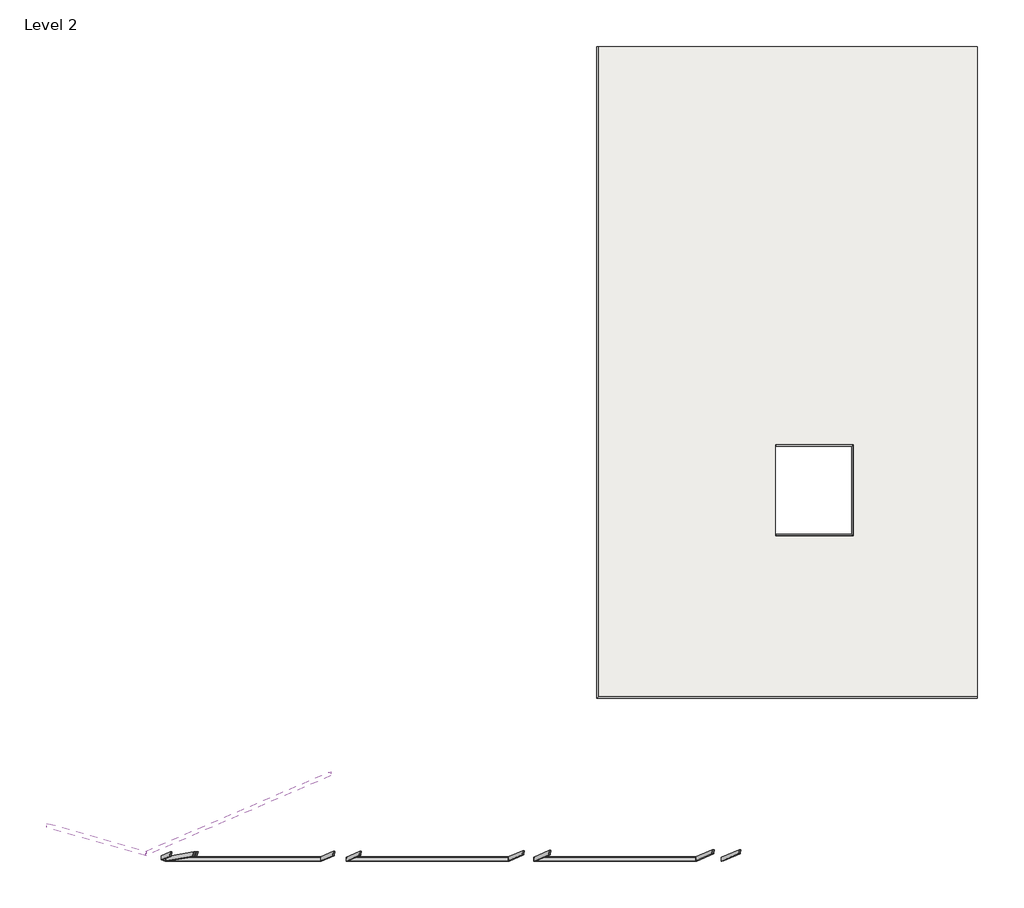
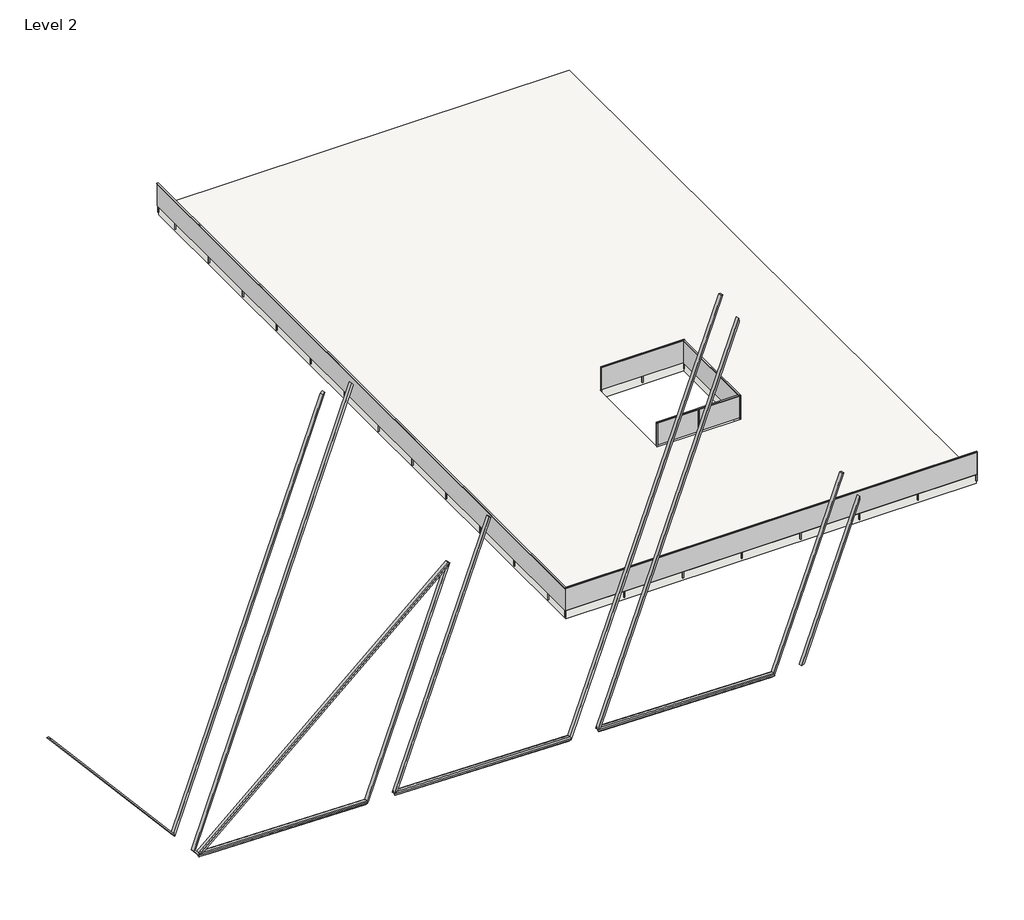
# One storey: 18 members, 2 railings, 1 slab.
"""IFC4 building model written with IfcOpenShell, lengths in millimetres."""

import ifcopenshell
import ifcopenshell.guid

model = None  # the IFC model being written
_history = None  # IfcOwnerHistory: only IFC2X3 demands one
_inside = {}  # id of a spatial element -> (the spatial element, [elements in it])
_under = {}  # id of a project, library or spatial element -> (it, [spatial elements below it])
_declared = {}  # id of a project -> (the project, [libraries it declares])
_typed = {}  # id of a type object -> (the type object, [elements of that type])
_made_of = {}  # id of a material, layer set ... -> (it, [elements and type objects made of it])


def new_model(schema):
    """Start an empty IFC model of exactly this schema.

    Asked for "IFC4X3", IfcOpenShell would pick the latest addendum, in which some entities
    have other attributes; the version numbers below select the first issue.
    IFC2X3 requires an IfcOwnerHistory on every rooted entity: one is made here for all.
    """
    global model, _history
    if schema == "IFC4X3":
        model = ifcopenshell.file(schema_version=(4, 3, 0, 0))
    else:
        model = ifcopenshell.file(schema=schema)
    _inside.clear()
    _under.clear()
    _declared.clear()
    _typed.clear()
    _made_of.clear()
    _history = None
    if model.schema == "IFC2X3":
        org = make("IfcOrganization", Name="unknown")
        user = make(
            "IfcPersonAndOrganization",
            ThePerson=make("IfcPerson", FamilyName="unknown"),
            TheOrganization=org,
        )
        app = make(
            "IfcApplication",
            ApplicationDeveloper=org,
            Version="unknown",
            ApplicationFullName="unknown",
            ApplicationIdentifier="unknown",
        )
        _history = make(
            "IfcOwnerHistory",
            OwningUser=user,
            OwningApplication=app,
            ChangeAction="ADDED",
            CreationDate=0,
        )
    return model


def make(cls, **values):
    """One entity of the class cls with the attributes given. An attribute that is None is left unset."""
    return model.create_entity(
        cls, **{name: value for name, value in values.items() if value is not None}
    )


def rooted(cls, **values):
    """An entity with a GlobalId (a new one), such as an element, a storey or a relation."""
    return make(cls, GlobalId=ifcopenshell.guid.new(), OwnerHistory=_history, **values)


def si_unit(unit_type, name, prefix=None):
    """IfcSIUnit, for example si_unit("LENGTHUNIT", "METRE", prefix="MILLI")."""
    return make("IfcSIUnit", UnitType=unit_type, Prefix=prefix, Name=name)


def assignment(units):
    """IfcUnitAssignment: the units of a project."""
    return None if units is None else make("IfcUnitAssignment", Units=units)


def point(xyz):
    """IfcCartesianPoint."""
    return None if xyz is None else make("IfcCartesianPoint", Coordinates=xyz)


def direction(xyz):
    """IfcDirection."""
    return None if xyz is None else make("IfcDirection", DirectionRatios=xyz)


def frame(location, z_axis=None, x_axis=None):
    """IfcAxis2Placement3D, a coordinate frame: its origin and axes. An axis left out is left unset."""
    return make(
        "IfcAxis2Placement3D",
        Location=point(location),
        Axis=direction(z_axis),
        RefDirection=direction(x_axis),
    )


def origin():
    """The frame at (0, 0, 0) with its axes left unset."""
    return frame((0.0, 0.0, 0.0))


def place(relative_to, where):
    """IfcLocalPlacement: puts the frame where relative to a parent placement (None: the world)."""
    return make(
        "IfcLocalPlacement", PlacementRelTo=relative_to, RelativePlacement=where
    )


def context(
    kind, dimensions, precision=None, world=None, true_north=None, identifier=None
):
    """IfcGeometricRepresentationContext, for example the 3D "Model" context."""
    return make(
        "IfcGeometricRepresentationContext",
        ContextIdentifier=identifier,
        ContextType=kind,
        CoordinateSpaceDimension=dimensions,
        Precision=precision,
        WorldCoordinateSystem=world,
        TrueNorth=true_north,
    )


def project(units=None, contexts=None):
    """IfcProject with its units and contexts."""
    return rooted(
        "IfcProject",
        Name="project",
        RepresentationContexts=contexts,
        UnitsInContext=assignment(units),
    )


def spatial(cls, under=None, at=None, **own):
    """A site, building, storey or space (cls), placed at a placement, below another one or the project."""
    s = rooted(cls, ObjectPlacement=at, **own)
    if under is not None:
        _under.setdefault(under.id(), (under, []))[1].append(s)
    return s


def polyline(points):
    """IfcPolyline through the points."""
    return make("IfcPolyline", Points=[point(p) for p in points])


def outline(outer, holes=None, kind="AREA"):
    """IfcArbitraryClosedProfileDef: a profile drawn as a closed curve; with holes, ...WithVoids."""
    if holes is None:
        return make("IfcArbitraryClosedProfileDef", ProfileType=kind, OuterCurve=outer)
    return make(
        "IfcArbitraryProfileDefWithVoids",
        ProfileType=kind,
        OuterCurve=outer,
        InnerCurves=holes,
    )


def extrude(swept, where, along, depth):
    """IfcExtrudedAreaSolid: the profile swept, set in the frame where, extruded along a direction by depth."""
    return make(
        "IfcExtrudedAreaSolid",
        SweptArea=swept,
        Position=where,
        ExtrudedDirection=direction(along),
        Depth=depth,
    )


def faces_of(points, faces, orient=None, outer=None):
    """IfcFace entities. A face is a list of loops; a loop is a list of indices into points, from 0.

    orient and outer hold one flag for each loop. By default every Orientation is true, the
    first loop of a face is its IfcFaceOuterBound and the others are IfcFaceBound.
    """
    made = []
    for i, loops in enumerate(faces):
        bounds = []
        for j, loop in enumerate(loops):
            is_outer = j == 0 if outer is None else outer[i][j]
            bounds.append(
                make(
                    "IfcFaceOuterBound" if is_outer else "IfcFaceBound",
                    Bound=make("IfcPolyLoop", Polygon=[points[k] for k in loop]),
                    Orientation=True if orient is None else orient[i][j],
                )
            )
        made.append(make("IfcFace", Bounds=bounds))
    return made


def faceted_brep(points, faces, orient=None, outer=None, voids=None):
    """IfcFacetedBrep: a solid bounded by flat faces; with voids (closed shells), ...WithVoids."""
    shared = [point(p) for p in points]
    hull = make("IfcClosedShell", CfsFaces=faces_of(shared, faces, orient, outer))
    if voids is None:
        return make("IfcFacetedBrep", Outer=hull)
    return make(
        "IfcFacetedBrepWithVoids",
        Outer=hull,
        Voids=[
            make(cls, CfsFaces=faces_of(shared, fs, o, b)) for cls, fs, o, b in voids
        ],
    )


def shape(context_of_items, identifier, shape_type, items):
    """IfcShapeRepresentation: the items that make up one representation, for example the "Body"."""
    return make(
        "IfcShapeRepresentation",
        ContextOfItems=context_of_items,
        RepresentationIdentifier=identifier,
        RepresentationType=shape_type,
        Items=items,
    )


def source(mapping_origin, context_of_items, identifier, shape_type, items):
    """IfcRepresentationMap: a shape defined once, which mapped items show again and again."""
    return make(
        "IfcRepresentationMap",
        MappingOrigin=mapping_origin,
        MappedRepresentation=shape(context_of_items, identifier, shape_type, items),
    )


def transform(
    local_origin,
    x_axis=None,
    y_axis=None,
    z_axis=None,
    scale=None,
    scale2=None,
    scale3=None,
    uniform=True,
):
    """IfcCartesianTransformationOperator3D, or its non-uniform kind. x_axis, y_axis, z_axis: its Axis1, 2, 3."""
    if uniform:
        return make(
            "IfcCartesianTransformationOperator3D",
            Axis1=direction(x_axis),
            Axis2=direction(y_axis),
            LocalOrigin=point(local_origin),
            Scale=scale,
            Axis3=direction(z_axis),
        )
    return make(
        "IfcCartesianTransformationOperator3DnonUniform",
        Axis1=direction(x_axis),
        Axis2=direction(y_axis),
        LocalOrigin=point(local_origin),
        Scale=scale,
        Axis3=direction(z_axis),
        Scale2=scale2,
        Scale3=scale3,
    )


def mapped(mapping_source, mapping_target):
    """IfcMappedItem: shows the shape of a source again, moved by a transform."""
    return make(
        "IfcMappedItem", MappingSource=mapping_source, MappingTarget=mapping_target
    )


def made_of(thing, what):
    """Note that an element or type object is made of a material, layer set ...; save() writes the relation."""
    if what is not None:
        _made_of.setdefault(what.id(), (what, []))[1].append(thing)
    return thing


def element(
    cls,
    number,
    at=None,
    inside=None,
    cuts=None,
    type_object=None,
    material=None,
    context=None,
    identifier="Body",
    shape_type=None,
    held_by="IfcProductDefinitionShape",
    body=None,
    shapes=None,
    **own,
):
    """One element of the class cls, such as IfcWall. Its Tag is "e" and its number.

    at: its placement. inside: the storey or other place that contains it. cuts: it is an
    opening in that element (IfcRelVoidsElement). A single representation is given by context,
    identifier, shape_type and body (its items); several are given by shapes. held_by: the class
    of the entity that holds the representations. save() writes the other relations.
    """
    e = rooted(cls, Tag="e%d" % number, ObjectPlacement=at, **own)
    if body is not None:
        shapes = [shape(context, identifier, shape_type, body)]
    if shapes is not None:
        e.Representation = make(held_by, Representations=shapes)
    if inside is not None:
        _inside.setdefault(inside.id(), (inside, []))[1].append(e)
    if cuts is not None:
        rooted(
            "IfcRelVoidsElement", RelatingBuildingElement=cuts, RelatedOpeningElement=e
        )
    if type_object is not None:
        _typed.setdefault(type_object.id(), (type_object, []))[1].append(e)
    return made_of(e, material)


def aggregate(whole, parts):
    """IfcRelAggregates: a whole, such as a stair, and the parts it consists of."""
    return rooted("IfcRelAggregates", RelatingObject=whole, RelatedObjects=parts)


def save(model, path):
    """Write the relations noted so far, then the file.

    IfcRelAggregates (storeys below a building ...), IfcRelContainedInSpatialStructure (elements
    in a storey), IfcRelDefinesByType, IfcRelAssociatesMaterial and IfcRelDeclares: one each for
    every whole, place, type object, material and project.
    """
    for whole, parts in _under.values():
        aggregate(whole, parts)
    for where, things in _inside.values():
        rooted(
            "IfcRelContainedInSpatialStructure",
            RelatedElements=things,
            RelatingStructure=where,
        )
    for kind, things in _typed.values():
        rooted("IfcRelDefinesByType", RelatedObjects=things, RelatingType=kind)
    for what, things in _made_of.values():
        rooted("IfcRelAssociatesMaterial", RelatedObjects=things, RelatingMaterial=what)
    for by, libraries in _declared.values():
        rooted("IfcRelDeclares", RelatingContext=by, RelatedDefinitions=libraries)
    model.write(path)


def rectangular_mullion_50_x_150mm_45e6ae42(model_context):
    return source(origin(), model_context, "Body", "SweptSolid", [
        extrude(outline(polyline([(0.0, 0.0), (-213.5028682, -50.0), (-7489.7328456, -50.0), (-7519.6193703, 0.0), (0.0, 0.0)])), frame((0.0, -75.0, 0.0), z_axis=(0.0, 1.0, 0.0), x_axis=(0.0, 0.0, 1.0)), (0.0, 0.0, 1.0), 150.0),
    ])


def rectangular_mullion_50_x_150mm_7bc3959f(model_context):
    return source(origin(), model_context, "Body", "SweptSolid", [
        extrude(outline(polyline([(0.0, 0.0), (-25.8377402, -50.0), (-13921.2143035, -50.0), (-13951.1008282, 0.0), (0.0, 0.0)])), frame((0.0, -75.0, 0.0), z_axis=(0.0, 1.0, 0.0), x_axis=(0.0, 0.0, 1.0)), (0.0, 0.0, 1.0), 150.0),
    ])


def rectangular_mullion_50_x_150mm_85ac93d7(model_context):
    return source(origin(), model_context, "Body", "SweptSolid", [
        extrude(outline(polyline([(0.0, 0.0), (-25.8377402, -50.0), (-6312.9528574, -50.0), (-6342.8393821, 0.0), (0.0, 0.0)])), frame((0.0, -75.0, 0.0), z_axis=(0.0, 1.0, 0.0), x_axis=(0.0, 0.0, 1.0)), (0.0, 0.0, 1.0), 150.0),
    ])


def rectangular_mullion_50_x_150mm_72219edf(model_context):
    return source(origin(), model_context, "Body", "SweptSolid", [
        extrude(outline(polyline([(0.0, 0.0), (-83.6497392, -50.0), (-5243.3853965, -50.0), (-5340.1430845, 0.0), (0.0, 0.0)])), frame((0.0, -75.0, 0.0), z_axis=(0.0, 1.0, 0.0), x_axis=(0.0, 0.0, 1.0)), (0.0, 0.0, 1.0), 150.0),
    ])


def rectangular_mullion_50_x_150mm_d07257d7(model_context):
    return source(origin(), model_context, "Body", "SweptSolid", [
        extrude(outline(polyline([(0.0, 0.0), (-83.6497392, -50.0), (-8698.3621073, -50.0), (-8710.0715519, 0.0), (0.0, 0.0)])), frame((0.0, -75.0, 0.0), z_axis=(0.0, 1.0, 0.0), x_axis=(0.0, 0.0, 1.0)), (0.0, 0.0, 1.0), 150.0),
    ])


def rectangular_mullion_50_x_150mm_06c78d0c(model_context):
    return source(origin(), model_context, "Body", "SweptSolid", [
        extrude(outline(polyline([(0.0, 0.0), (-83.6497392, -50.0), (-12851.6468426, -50.0), (-12948.4045305, 0.0), (0.0, 0.0)])), frame((0.0, -75.0, 0.0), z_axis=(0.0, 1.0, 0.0), x_axis=(0.0, 0.0, 1.0)), (0.0, 0.0, 1.0), 150.0),
    ])


def rectangular_mullion_50_x_150mm_e862281f(model_context):
    return source(origin(), model_context, "Body", "SweptSolid", [
        extrude(outline(polyline([(0.0, 0.0), (-85.321119, -50.0), (-13880.4605319, -50.0), (-13952.0824058, 0.0), (0.0, 0.0)])), frame((0.0, -75.0, 0.0), z_axis=(0.0, 1.0, 0.0), x_axis=(0.0, 0.0, 1.0)), (0.0, 0.0, 1.0), 150.0),
    ])


def rectangular_mullion_50_x_150mm_72e471df(model_context):
    return source(origin(), model_context, "Body", "SweptSolid", [
        extrude(outline(polyline([(0.0, 0.0), (-34.9055374, -50.0), (-14669.1673585, -50.0), (-14698.4684276, 0.0), (0.0, 0.0)])), frame((0.0, -75.0, 0.0), z_axis=(0.0, 1.0, 0.0), x_axis=(0.0, 0.0, 1.0)), (0.0, 0.0, 1.0), 150.0),
    ])


def rectangular_mullion_50_x_150mm_2c60866a(model_context):
    return source(origin(), model_context, "Body", "SweptSolid", [
        extrude(outline(polyline([(0.0, 0.0), (-71.6218739, -50.0), (-5613.3621531, -50.0), (-5648.2676905, 0.0), (0.0, 0.0)])), frame((0.0, -75.0, 0.0), z_axis=(0.0, 1.0, 0.0), x_axis=(0.0, 0.0, 1.0)), (0.0, 0.0, 1.0), 150.0),
    ])


def rectangular_mullion_50_x_150mm_55f3bd26(model_context):
    return source(origin(), model_context, "Body", "SweptSolid", [
        extrude(outline(polyline([(0.0, 0.0), (-44.8446171, -50.0), (-197.6121942, -50.0), (-232.5177317, 0.0), (0.0, 0.0)])), frame((0.0, -75.0, 0.0), z_axis=(0.0, 1.0, 0.0), x_axis=(0.0, 0.0, 1.0)), (0.0, 0.0, 1.0), 150.0),
    ])


def rectangular_mullion_50_x_150mm_04a9887f(model_context):
    return source(origin(), model_context, "Body", "SweptSolid", [
        extrude(outline(polyline([(0.0, 0.0), (-29.8865247, -50.0), (-5610.6120574, -50.0), (-5767.4004184, 0.0), (0.0, 0.0)])), frame((0.0, -75.0, 0.0), z_axis=(0.0, 1.0, 0.0), x_axis=(0.0, 0.0, 1.0)), (0.0, 0.0, 1.0), 150.0),
    ])


def rectangular_mullion_50_x_150mm_9d0fdde0(model_context):
    return source(origin(), model_context, "Body", "SweptSolid", [
        extrude(outline(polyline([(0.0, 0.0), (-29.8865247, -50.0), (-5931.3660368, -50.0), (-6015.015776, 0.0), (0.0, 0.0)])), frame((0.0, -75.0, 0.0), z_axis=(0.0, 1.0, 0.0), x_axis=(0.0, 0.0, 1.0)), (0.0, 0.0, 1.0), 150.0),
    ])


def rectangular_mullion_50_x_150mm_26c19414(model_context):
    return source(origin(), model_context, "Body", "SweptSolid", [
        extrude(outline(polyline([(0.0, 0.0), (-156.788361, -50.0), (-11226.8029982, -50.0), (-11440.3058664, 0.0), (0.0, 0.0)])), frame((0.0, -75.0, 0.0), z_axis=(0.0, 1.0, 0.0), x_axis=(0.0, 0.0, 1.0)), (0.0, 0.0, 1.0), 150.0),
    ])


def rectangular_mullion_50_x_150mm_985ce2fd(model_context):
    return source(origin(), model_context, "Body", "SweptSolid", [
        extrude(outline(polyline([(0.0, 0.0), (-11.7200342, -50.0), (-11395.4612493, -50.0), (-11440.3058664, 0.0), (0.0, 0.0)])), frame((0.0, -75.0, 0.0), z_axis=(0.0, 1.0, 0.0), x_axis=(0.0, 0.0, 1.0)), (0.0, 0.0, 1.0), 150.0),
    ])


def rectangular_mullion_50_x_150mm_1c2bc1f0(model_context):
    return source(origin(), model_context, "Body", "SweptSolid", [
        extrude(outline(polyline([(0.0, 0.0), (-433.116945, -50.0), (-5688.9606912, -50.0), (-5767.4004184, 0.0), (0.0, 0.0)])), frame((0.0, -75.0, 0.0), z_axis=(0.0, 1.0, 0.0), x_axis=(0.0, 0.0, 1.0)), (0.0, 0.0, 1.0), 150.0),
    ])


def rectangular_mullion_50_x_150mm_abaa279f(model_context):
    return source(origin(), model_context, "Body", "SweptSolid", [
        extrude(outline(polyline([(0.0, 0.0), (-31.871605, -50.0), (-5936.5760489, -50.0), (-6015.015776, 0.0), (0.0, 0.0)])), frame((0.0, -75.0, 0.0), z_axis=(0.0, 1.0, 0.0), x_axis=(0.0, 0.0, 1.0)), (0.0, 0.0, 1.0), 150.0),
    ])


def glas_mpk_99f97afc(model_context):
    return source(origin(), model_context, "Body", "SolidModel", [
        faceted_brep([(22257.9971367, 15998.757723, 3843.2628643), (22207.9971367, 15998.757723, 3843.2628643), (22207.9971367, 15998.757723, 3856.7371357), (22257.9971367, 15998.757723, 3856.7371357), (36243.4971367, -8011.242277, 3843.2628643), (36243.4971367, -8011.242277, 3856.7371357), (36243.4971367, -8061.242277, 3856.7371357), (36243.4971367, -8061.242277, 3843.2628643), (22257.9971367, -8011.242277, 3843.2628643), (22207.9971367, -8061.242277, 3843.2628643), (22207.9971367, -8061.242277, 3856.7371357), (22257.9971367, -8011.242277, 3856.7371357)], [[[0, 1, 2, 3]], [[4, 5, 6, 7]], [[1, 0, 8, 9]], [[2, 1, 9, 10]], [[3, 2, 10, 11]], [[0, 3, 11, 8]], [[9, 8, 4, 7]], [[10, 9, 7, 6]], [[11, 10, 6, 5]], [[8, 11, 5, 4]]]),
        faceted_brep([(22217.9971367, 15998.757723, 3842.8769824), (22232.1892606, 15998.757723, 3842.8769824), (22232.1892606, 15998.757723, 3042.8769824), (22217.9971367, 15998.757723, 3042.8769824), (22217.9971367, -8051.242277, 3842.8769824), (22232.1892606, -8037.0501531, 3842.8769824), (22232.1892606, -8037.0501531, 3042.8769824), (22217.9971367, -8051.242277, 3042.8769824), (36243.4971367, -8051.242277, 3842.8769824), (36243.4971367, -8051.242277, 3042.8769824), (36243.4971367, -8037.0501531, 3042.8769824), (36243.4971367, -8037.0501531, 3842.8769824)], [[[0, 1, 2, 3]], [[1, 0, 4, 5]], [[2, 1, 5, 6]], [[3, 2, 6, 7]], [[0, 3, 7, 4]], [[8, 9, 10, 11]], [[5, 4, 8, 11]], [[6, 5, 11, 10]], [[7, 6, 10, 9]], [[4, 7, 9, 8]]]),
        extrude(outline(polyline([(34236.9971367, -8036.242277), (34236.9971367, -8011.242277), (34261.9971367, -8011.242277), (34261.9971367, -8036.242277), (34236.9971367, -8036.242277)])), frame((0.0, 0.0, 2800.0), z_axis=(0.0, 0.0, 1.0), x_axis=(1.0, 0.0, 0.0)), (0.0, 0.0, 1.0), 1043.2628643),
        extrude(outline(polyline([(32236.9971367, -8036.242277), (32236.9971367, -8011.242277), (32261.9971367, -8011.242277), (32261.9971367, -8036.242277), (32236.9971367, -8036.242277)])), frame((0.0, 0.0, 2800.0), z_axis=(0.0, 0.0, 1.0), x_axis=(1.0, 0.0, 0.0)), (0.0, 0.0, 1.0), 1043.2628643),
        extrude(outline(polyline([(30236.9971367, -8036.242277), (30236.9971367, -8011.242277), (30261.9971367, -8011.242277), (30261.9971367, -8036.242277), (30236.9971367, -8036.242277)])), frame((0.0, 0.0, 2800.0), z_axis=(0.0, 0.0, 1.0), x_axis=(1.0, 0.0, 0.0)), (0.0, 0.0, 1.0), 1043.2628643),
        extrude(outline(polyline([(28236.9971367, -8036.242277), (28236.9971367, -8011.242277), (28261.9971367, -8011.242277), (28261.9971367, -8036.242277), (28236.9971367, -8036.242277)])), frame((0.0, 0.0, 2800.0), z_axis=(0.0, 0.0, 1.0), x_axis=(1.0, 0.0, 0.0)), (0.0, 0.0, 1.0), 1043.2628643),
        extrude(outline(polyline([(26236.9971367, -8036.242277), (26236.9971367, -8011.242277), (26261.9971367, -8011.242277), (26261.9971367, -8036.242277), (26236.9971367, -8036.242277)])), frame((0.0, 0.0, 2800.0), z_axis=(0.0, 0.0, 1.0), x_axis=(1.0, 0.0, 0.0)), (0.0, 0.0, 1.0), 1043.2628643),
        extrude(outline(polyline([(24236.9971367, -8036.242277), (24236.9971367, -8011.242277), (24261.9971367, -8011.242277), (24261.9971367, -8036.242277), (24236.9971367, -8036.242277)])), frame((0.0, 0.0, 2800.0), z_axis=(0.0, 0.0, 1.0), x_axis=(1.0, 0.0, 0.0)), (0.0, 0.0, 1.0), 1043.2628643),
        extrude(outline(polyline([(22232.9971367, -6994.992277), (22257.9971367, -6994.992277), (22257.9971367, -7019.992277), (22232.9971367, -7019.992277), (22232.9971367, -6994.992277)])), frame((0.0, 0.0, 2800.0), z_axis=(0.0, 0.0, 1.0), x_axis=(1.0, 0.0, 0.0)), (0.0, 0.0, 1.0), 1043.2628643),
        extrude(outline(polyline([(22232.9971367, -4994.992277), (22257.9971367, -4994.992277), (22257.9971367, -5019.992277), (22232.9971367, -5019.992277), (22232.9971367, -4994.992277)])), frame((0.0, 0.0, 2800.0), z_axis=(0.0, 0.0, 1.0), x_axis=(1.0, 0.0, 0.0)), (0.0, 0.0, 1.0), 1043.2628643),
        extrude(outline(polyline([(22232.9971367, -2994.992277), (22257.9971367, -2994.992277), (22257.9971367, -3019.992277), (22232.9971367, -3019.992277), (22232.9971367, -2994.992277)])), frame((0.0, 0.0, 2800.0), z_axis=(0.0, 0.0, 1.0), x_axis=(1.0, 0.0, 0.0)), (0.0, 0.0, 1.0), 1043.2628643),
        extrude(outline(polyline([(22232.9971367, -994.992277), (22257.9971367, -994.992277), (22257.9971367, -1019.992277), (22232.9971367, -1019.992277), (22232.9971367, -994.992277)])), frame((0.0, 0.0, 2800.0), z_axis=(0.0, 0.0, 1.0), x_axis=(1.0, 0.0, 0.0)), (0.0, 0.0, 1.0), 1043.2628643),
        extrude(outline(polyline([(22232.9971367, 1005.007723), (22257.9971367, 1005.007723), (22257.9971367, 980.007723), (22232.9971367, 980.007723), (22232.9971367, 1005.007723)])), frame((0.0, 0.0, 2800.0), z_axis=(0.0, 0.0, 1.0), x_axis=(1.0, 0.0, 0.0)), (0.0, 0.0, 1.0), 1043.2628643),
        extrude(outline(polyline([(22232.9971367, 3005.007723), (22257.9971367, 3005.007723), (22257.9971367, 2980.007723), (22232.9971367, 2980.007723), (22232.9971367, 3005.007723)])), frame((0.0, 0.0, 2800.0), z_axis=(0.0, 0.0, 1.0), x_axis=(1.0, 0.0, 0.0)), (0.0, 0.0, 1.0), 1043.2628643),
        extrude(outline(polyline([(22232.9971367, 5005.007723), (22257.9971367, 5005.007723), (22257.9971367, 4980.007723), (22232.9971367, 4980.007723), (22232.9971367, 5005.007723)])), frame((0.0, 0.0, 2800.0), z_axis=(0.0, 0.0, 1.0), x_axis=(1.0, 0.0, 0.0)), (0.0, 0.0, 1.0), 1043.2628643),
        extrude(outline(polyline([(22232.9971367, 7005.007723), (22257.9971367, 7005.007723), (22257.9971367, 6980.007723), (22232.9971367, 6980.007723), (22232.9971367, 7005.007723)])), frame((0.0, 0.0, 2800.0), z_axis=(0.0, 0.0, 1.0), x_axis=(1.0, 0.0, 0.0)), (0.0, 0.0, 1.0), 1043.2628643),
        extrude(outline(polyline([(22232.9971367, 9005.007723), (22257.9971367, 9005.007723), (22257.9971367, 8980.007723), (22232.9971367, 8980.007723), (22232.9971367, 9005.007723)])), frame((0.0, 0.0, 2800.0), z_axis=(0.0, 0.0, 1.0), x_axis=(1.0, 0.0, 0.0)), (0.0, 0.0, 1.0), 1043.2628643),
        extrude(outline(polyline([(22232.9971367, 11005.007723), (22257.9971367, 11005.007723), (22257.9971367, 10980.007723), (22232.9971367, 10980.007723), (22232.9971367, 11005.007723)])), frame((0.0, 0.0, 2800.0), z_axis=(0.0, 0.0, 1.0), x_axis=(1.0, 0.0, 0.0)), (0.0, 0.0, 1.0), 1043.2628643),
        extrude(outline(polyline([(22232.9971367, 13005.007723), (22257.9971367, 13005.007723), (22257.9971367, 12980.007723), (22232.9971367, 12980.007723), (22232.9971367, 13005.007723)])), frame((0.0, 0.0, 2800.0), z_axis=(0.0, 0.0, 1.0), x_axis=(1.0, 0.0, 0.0)), (0.0, 0.0, 1.0), 1043.2628643),
        extrude(outline(polyline([(22232.9971367, 15005.007723), (22257.9971367, 15005.007723), (22257.9971367, 14980.007723), (22232.9971367, 14980.007723), (22232.9971367, 15005.007723)])), frame((0.0, 0.0, 2800.0), z_axis=(0.0, 0.0, 1.0), x_axis=(1.0, 0.0, 0.0)), (0.0, 0.0, 1.0), 1043.2628643),
        extrude(outline(polyline([(22232.9971367, -8001.242277), (22257.9971367, -8001.242277), (22257.9971367, -8026.242277), (22232.9971367, -8026.242277), (22232.9971367, -8001.242277)])), frame((0.0, 0.0, 2800.0), z_axis=(0.0, 0.0, 1.0), x_axis=(1.0, 0.0, 0.0)), (0.0, 0.0, 1.0), 1043.2628643),
        extrude(outline(polyline([(36230.9971367, -8036.242277), (36230.9971367, -8011.242277), (36255.9971367, -8011.242277), (36255.9971367, -8036.242277), (36230.9971367, -8036.242277)])), frame((0.0, 0.0, 2800.0), z_axis=(0.0, 0.0, 1.0), x_axis=(1.0, 0.0, 0.0)), (0.0, 0.0, 1.0), 1043.2628643),
        extrude(outline(polyline([(22232.9971367, 15998.757723), (22257.9971367, 15998.757723), (22257.9971367, 15973.757723), (22232.9971367, 15973.757723), (22232.9971367, 15998.757723)])), frame((0.0, 0.0, 2800.0), z_axis=(0.0, 0.0, 1.0), x_axis=(1.0, 0.0, 0.0)), (0.0, 0.0, 1.0), 1043.2628643),
    ])


def glas_mpk_050cb379(model_context):
    return source(origin(), model_context, "Body", "SolidModel", [
        faceted_brep([(28820.3199184, 1288.5335867, 3843.2628643), (28820.3199184, 1238.5335867, 3843.2628643), (28820.3199184, 1238.5335867, 3856.7371357), (28820.3199184, 1288.5335867, 3856.7371357), (31660.3199184, 1288.5335867, 3843.2628643), (31610.3199184, 1238.5335867, 3843.2628643), (31610.3199184, 1238.5335867, 3856.7371357), (31660.3199184, 1288.5335867, 3856.7371357), (31660.3199184, -2052.1957594, 3843.2628643), (31610.3199184, -2002.1957594, 3843.2628643), (31610.3199184, -2002.1957594, 3856.7371357), (31660.3199184, -2052.1957594, 3856.7371357), (28820.3199184, -2052.1957594, 3843.2628643), (28820.3199184, -2052.1957594, 3856.7371357), (28820.3199184, -2002.1957594, 3856.7371357), (28820.3199184, -2002.1957594, 3843.2628643)], [[[0, 1, 2, 3]], [[1, 0, 4, 5]], [[2, 1, 5, 6]], [[3, 2, 6, 7]], [[0, 3, 7, 4]], [[5, 4, 8, 9]], [[6, 5, 9, 10]], [[7, 6, 10, 11]], [[4, 7, 11, 8]], [[12, 13, 14, 15]], [[9, 8, 12, 15]], [[10, 9, 15, 14]], [[11, 10, 14, 13]], [[8, 11, 13, 12]]]),
        faceted_brep([(28820.3199184, 1248.5335867, 3842.8769824), (28820.3199184, 1262.7257107, 3842.8769824), (28820.3199184, 1262.7257107, 3042.8769824), (28820.3199184, 1248.5335867, 3042.8769824), (31620.3199184, 1248.5335867, 3842.8769824), (31634.5120424, 1262.7257107, 3842.8769824), (31634.5120424, 1262.7257107, 3042.8769824), (31620.3199184, 1248.5335867, 3042.8769824), (31620.3199184, -2012.1957594, 3842.8769824), (31634.5120424, -2026.3878834, 3842.8769824), (31634.5120424, -2026.3878834, 3042.8769824), (31620.3199184, -2012.1957594, 3042.8769824), (28820.3199184, -2012.1957594, 3842.8769824), (28820.3199184, -2012.1957594, 3042.8769824), (28820.3199184, -2026.3878834, 3042.8769824), (28820.3199184, -2026.3878834, 3842.8769824)], [[[0, 1, 2, 3]], [[1, 0, 4, 5]], [[2, 1, 5, 6]], [[3, 2, 6, 7]], [[0, 3, 7, 4]], [[5, 4, 8, 9]], [[6, 5, 9, 10]], [[7, 6, 10, 11]], [[4, 7, 11, 8]], [[12, 13, 14, 15]], [[9, 8, 12, 15]], [[10, 9, 15, 14]], [[11, 10, 14, 13]], [[8, 11, 13, 12]]]),
        extrude(outline(polyline([(30251.5699184, -2027.1957594), (30251.5699184, -2052.1957594), (30226.5699184, -2052.1957594), (30226.5699184, -2027.1957594), (30251.5699184, -2027.1957594)])), frame((0.0, 0.0, 2800.0), z_axis=(0.0, 0.0, 1.0), x_axis=(1.0, 0.0, 0.0)), (0.0, 0.0, 1.0), 1043.2628643),
        extrude(outline(polyline([(31635.3199184, -369.3310864), (31660.3199184, -369.3310864), (31660.3199184, -394.3310864), (31635.3199184, -394.3310864), (31635.3199184, -369.3310864)])), frame((0.0, 0.0, 2800.0), z_axis=(0.0, 0.0, 1.0), x_axis=(1.0, 0.0, 0.0)), (0.0, 0.0, 1.0), 1043.2628643),
        extrude(outline(polyline([(30226.5699184, 1263.5335867), (30226.5699184, 1288.5335867), (30251.5699184, 1288.5335867), (30251.5699184, 1263.5335867), (30226.5699184, 1263.5335867)])), frame((0.0, 0.0, 2800.0), z_axis=(0.0, 0.0, 1.0), x_axis=(1.0, 0.0, 0.0)), (0.0, 0.0, 1.0), 1043.2628643),
        extrude(outline(polyline([(31635.3199184, -2037.1957594), (31660.3199184, -2037.1957594), (31660.3199184, -2062.1957594), (31635.3199184, -2062.1957594), (31635.3199184, -2037.1957594)])), frame((0.0, 0.0, 2800.0), z_axis=(0.0, 0.0, 1.0), x_axis=(1.0, 0.0, 0.0)), (0.0, 0.0, 1.0), 1043.2628643),
        extrude(outline(polyline([(31645.3199184, 1263.5335867), (31645.3199184, 1288.5335867), (31670.3199184, 1288.5335867), (31670.3199184, 1263.5335867), (31645.3199184, 1263.5335867)])), frame((0.0, 0.0, 2800.0), z_axis=(0.0, 0.0, 1.0), x_axis=(1.0, 0.0, 0.0)), (0.0, 0.0, 1.0), 1043.2628643),
        extrude(outline(polyline([(28832.8199184, -2027.1957594), (28832.8199184, -2052.1957594), (28807.8199184, -2052.1957594), (28807.8199184, -2027.1957594), (28832.8199184, -2027.1957594)])), frame((0.0, 0.0, 2800.0), z_axis=(0.0, 0.0, 1.0), x_axis=(1.0, 0.0, 0.0)), (0.0, 0.0, 1.0), 1043.2628643),
        extrude(outline(polyline([(28820.3199184, 1263.5335867), (28820.3199184, 1288.5335867), (28845.3199184, 1288.5335867), (28845.3199184, 1263.5335867), (28820.3199184, 1263.5335867)])), frame((0.0, 0.0, 2800.0), z_axis=(0.0, 0.0, 1.0), x_axis=(1.0, 0.0, 0.0)), (0.0, 0.0, 1.0), 1043.2628643),
    ])


model = new_model("IFC4")

# Units and contexts
model_context = context("Model", 3, world=origin())
ifc_project = project(units=[si_unit("LENGTHUNIT", "METRE", prefix="MILLI")], contexts=[model_context])

# Site, building, storey
site = spatial("IfcSite", under=ifc_project)
building = spatial("IfcBuilding", under=site)
storey = spatial("IfcBuildingStorey", under=building, Name="Level 2", Elevation=3000.0)

# Members
placement = place(None, origin())
rectangular_mullion_50_x_150mm_shape = rectangular_mullion_50_x_150mm_45e6ae42(model_context)
element("IfcMember", 1, ObjectType="Rectangular Mullion : 50 x 150mm", at=placement, inside=storey, context=model_context, shape_type="MappedRepresentation", body=[
    mapped(rectangular_mullion_50_x_150mm_shape, transform((15712.2362266, -12439.2631776, 9728.8576057), x_axis=(0.8722203744850089, -0.11167721831800664, -0.47619304619238534), y_axis=(-0.004309282844984025, 0.9717923608297845, -0.2357987224609922), z_axis=(0.489094109977408, 0.2077205005328708, 0.847135848163552))),
])
rectangular_mullion_50_x_150mm_2_shape = rectangular_mullion_50_x_150mm_7bc3959f(model_context)
element("IfcMember", 2, ObjectType="Rectangular Mullion : 50 x 150mm", at=placement, inside=storey, context=model_context, shape_type="MappedRepresentation", body=[
    mapped(rectangular_mullion_50_x_150mm_2_shape, transform((25784.748506, -11103.31263, 15050.6049804), x_axis=(0.8722203744850084, -0.1116772183180068, -0.476193046192386), y_axis=(-0.004309282844984081, 0.9717923608297845, -0.2357987224609923), z_axis=(0.48909410997740865, 0.2077205005328708, 0.8471358481635516))),
])
rectangular_mullion_50_x_150mm_3_shape = rectangular_mullion_50_x_150mm_85ac93d7(model_context)
element("IfcMember", 3, ObjectType="Rectangular Mullion : 50 x 150mm", at=placement, inside=storey, context=model_context, shape_type="MappedRepresentation", body=[
    mapped(rectangular_mullion_50_x_150mm_3_shape, transform((28990.5052254, -12683.7045058, 8478.7828423), x_axis=(0.872220374485008, -0.111677218318007, -0.4761930461923868), y_axis=(-0.0043092828449840664, 0.9717923608297845, -0.23579872246099232), z_axis=(0.48909410997740954, 0.20772050053287072, 0.8471358481635513))),
])
rectangular_mullion_50_x_150mm_4_shape = rectangular_mullion_50_x_150mm_72219edf(model_context)
element("IfcMember", 4, ObjectType="Rectangular Mullion : 50 x 150mm", at=placement, inside=storey, context=model_context, shape_type="MappedRepresentation", body=[
    mapped(rectangular_mullion_50_x_150mm_4_shape, transform((26801.1608583, -14001.242277, 3088.8527196), x_axis=(-0.8722203744850093, 0.11167721831800645, 0.47619304619238456), y_axis=(-0.004309282844983942, 0.9717923608297845, -0.23579872246099207), z_axis=(-0.48909410997740715, -0.20772050053287072, -0.8471358481635525))),
])
rectangular_mullion_50_x_150mm_5_shape = rectangular_mullion_50_x_150mm_d07257d7(model_context)
element("IfcMember", 5, ObjectType="Rectangular Mullion : 50 x 150mm", at=placement, inside=storey, context=model_context, shape_type="MappedRepresentation", body=[
    mapped(rectangular_mullion_50_x_150mm_5_shape, transform((12947.3356985, -14001.242277, 3342.0349696), x_axis=(-0.8722203744850089, 0.11167721831800664, 0.47619304619238534), y_axis=(-0.004309282844984094, 0.9717923608297845, -0.23579872246099232), z_axis=(-0.489094109977408, -0.20772050053287094, -0.847135848163552))),
])
rectangular_mullion_50_x_150mm_6_shape = rectangular_mullion_50_x_150mm_06c78d0c(model_context)
element("IfcMember", 6, ObjectType="Rectangular Mullion : 50 x 150mm", at=placement, inside=storey, context=model_context, shape_type="MappedRepresentation", body=[
    mapped(rectangular_mullion_50_x_150mm_6_shape, transform((19874.2482784, -14001.242277, 3215.4438446), x_axis=(-0.8722203744850086, 0.11167721831800675, 0.47619304619238584), y_axis=(-0.004309282844984137, 0.9717923608297845, -0.23579872246099243), z_axis=(-0.4890941099774085, -0.20772050053287094, -0.8471358481635517))),
])
rectangular_mullion_50_x_150mm_7_shape = rectangular_mullion_50_x_150mm_e862281f(model_context)
element("IfcMember", 7, ObjectType="Rectangular Mullion : 50 x 150mm", at=placement, inside=storey, context=model_context, shape_type="MappedRepresentation", body=[
    mapped(rectangular_mullion_50_x_150mm_7_shape, transform((12377.8841529, -10856.2576342, 16077.9460567), x_axis=(0.8724314351462177, -0.11823606660145627, -0.4742189615813851), y_axis=(0.0, 0.9702957262759964, -0.24192189559966842), z_axis=(0.4887365251019318, 0.211060266571311, 0.8465164929912092))),
])
rectangular_mullion_50_x_150mm_8_shape = rectangular_mullion_50_x_150mm_72e471df(model_context)
element("IfcMember", 8, ObjectType="Rectangular Mullion : 50 x 150mm", at=placement, inside=storey, context=model_context, shape_type="MappedRepresentation", body=[
    mapped(rectangular_mullion_50_x_150mm_8_shape, transform((6116.7390094, -13958.5202987, 3635.4501111), x_axis=(-0.8724314351462176, 0.11823606660145626, 0.47421896158138505), y_axis=(0.0, 0.9702957262759963, -0.24192189559966853), z_axis=(-0.4887365251019317, -0.21106026657131116, -0.8465164929912091))),
])
rectangular_mullion_50_x_150mm_9_shape = rectangular_mullion_50_x_150mm_2c60866a(model_context)
element("IfcMember", 9, ObjectType="Rectangular Mullion : 50 x 150mm", at=placement, inside=storey, context=model_context, shape_type="MappedRepresentation", body=[
    mapped(rectangular_mullion_50_x_150mm_9_shape, transform((5558.99188, -13800.987866, 4267.2781887), x_axis=(-0.7594865733990561, -0.15737575195413048, -0.6311996653384983), y_axis=(0.0, 0.9702957262759964, -0.2419218955996686), z_axis=(0.6505229779389504, -0.18373643151919805, -0.7369265763331045))),
])
rectangular_mullion_50_x_150mm_10_shape = rectangular_mullion_50_x_150mm_55f3bd26(model_context)
element("IfcMember", 10, ObjectType="Rectangular Mullion : 50 x 150mm", at=placement, inside=storey, context=model_context, shape_type="MappedRepresentation", body=[
    mapped(rectangular_mullion_50_x_150mm_10_shape, transform((6267.9971367, -14001.242277, 3464.1016151), x_axis=(-0.7594865733990622, -0.15737575195412876, -0.6311996653384914), y_axis=(0.0, 0.9702957262759964, -0.24192189559966823), z_axis=(0.6505229779389433, -0.183736431519199, -0.7369265763331105))),
])
rectangular_mullion_50_x_150mm_11_shape = rectangular_mullion_50_x_150mm_04a9887f(model_context)
element("IfcMember", 11, ObjectType="Rectangular Mullion : 50 x 150mm", at=placement, inside=storey, context=model_context, shape_type="MappedRepresentation", body=[
    mapped(rectangular_mullion_50_x_150mm_11_shape, transform((12034.4346833, -14001.242277, 3358.7184725), x_axis=(-0.017756792578909553, -0.23583809580488502, -0.9716301193789926), y_axis=(-0.00430928284498418, 0.9717923608297845, -0.23579872246099226), z_axis=(0.9998330492630614, 0.0, -0.018272208441469037))),
])
rectangular_mullion_50_x_150mm_12_shape = rectangular_mullion_50_x_150mm_9d0fdde0(model_context)
element("IfcMember", 12, ObjectType="Rectangular Mullion : 50 x 150mm", at=placement, inside=storey, context=model_context, shape_type="MappedRepresentation", body=[
    mapped(rectangular_mullion_50_x_150mm_12_shape, transform((18961.3472632, -14001.242277, 3232.1273475), x_axis=(-0.01775679257890959, -0.23583809580488502, -0.9716301193789926), y_axis=(-0.004309282844983898, 0.9717923608297845, -0.23579872246099226), z_axis=(0.9998330492630614, 0.0, -0.018272208441469005))),
])
element("IfcMember", 13, ObjectType="Rectangular Mullion : 50 x 150mm", at=placement, inside=storey, context=model_context, shape_type="MappedRepresentation", body=[
    mapped(rectangular_mullion_50_x_150mm_12_shape, transform((25888.2598431, -14001.242277, 3105.5362225), x_axis=(-0.01775679257890941, -0.23583809580488502, -0.9716301193789926), y_axis=(-0.004309282844984225, 0.9717923608297845, -0.23579872246099226), z_axis=(0.9998330492630614, 0.0, -0.01827220844146891))),
])
rectangular_mullion_50_x_150mm_13_shape = rectangular_mullion_50_x_150mm_26c19414(model_context)
element("IfcMember", 14, ObjectType="Rectangular Mullion : 50 x 150mm", at=placement, inside=storey, context=model_context, shape_type="MappedRepresentation", body=[
    mapped(rectangular_mullion_50_x_150mm_13_shape, transform((6267.9971367, -14001.242277, 3464.1016151), x_axis=(-0.5643515799010996, 0.19229756024024106, 0.8028255991115278), y_axis=(-0.0043092828449839415, 0.9717923608297845, -0.2357987224609922), z_axis=(-0.8255233033321923, -0.13653298414128712, -0.5476038895926328))),
])
rectangular_mullion_50_x_150mm_14_shape = rectangular_mullion_50_x_150mm_985ce2fd(model_context)
element("IfcMember", 15, ObjectType="Rectangular Mullion : 50 x 150mm", at=placement, inside=storey, context=model_context, shape_type="MappedRepresentation", body=[
    mapped(rectangular_mullion_50_x_150mm_14_shape, transform((15712.2362266, -12439.2631776, 9728.8576057), x_axis=(0.5643680320991838, -0.19971216240382536, -0.8010017331644688), y_axis=(0.0, 0.9702957262759964, -0.24192189559966845), z_axis=(0.8255233033321923, 0.13653298414128712, 0.5476038895926328))),
])
rectangular_mullion_50_x_150mm_15_shape = rectangular_mullion_50_x_150mm_1c2bc1f0(model_context)
element("IfcMember", 16, ObjectType="Rectangular Mullion : 50 x 150mm", at=placement, inside=storey, context=model_context, shape_type="MappedRepresentation", body=[
    mapped(rectangular_mullion_50_x_150mm_15_shape, transform((6267.9971367, -14001.242277, 3464.1016151), x_axis=(0.015380413782729804, -0.5398860921808011, 0.8415975584218478), y_axis=(0.009864911210979758, 0.8417380872158177, 0.5397959577998486), z_axis=(-0.9998330492630614, 0.0, 0.01827220844146922))),
])
rectangular_mullion_50_x_150mm_16_shape = rectangular_mullion_50_x_150mm_abaa279f(model_context)
element("IfcMember", 17, ObjectType="Rectangular Mullion : 50 x 150mm", at=placement, inside=storey, context=model_context, shape_type="MappedRepresentation", body=[
    mapped(rectangular_mullion_50_x_150mm_16_shape, transform((12947.3356985, -14001.242277, 3342.0349696), x_axis=(0.015380413782729674, -0.5398860921808011, 0.8415975584218478), y_axis=(0.009864911210979564, 0.8417380872158177, 0.5397959577998486), z_axis=(-0.9998330492630614, 0.0, 0.018272208441469005))),
])
element("IfcMember", 18, ObjectType="Rectangular Mullion : 50 x 150mm", at=placement, inside=storey, context=model_context, shape_type="MappedRepresentation", body=[
    mapped(rectangular_mullion_50_x_150mm_16_shape, transform((19874.2482784, -14001.242277, 3215.4438446), x_axis=(0.015380413782729887, -0.5398860921808011, 0.8415975584218478), y_axis=(0.009864911210979701, 0.8417380872158177, 0.5397959577998486), z_axis=(-0.9998330492630614, 0.0, 0.01827220844146926))),
])

# Railings
glas_mpk_shape = glas_mpk_99f97afc(model_context)
element("IfcRailing", 19, ObjectType="Glas - MPK", at=placement, inside=storey, context=model_context, shape_type="MappedRepresentation", body=[
    mapped(glas_mpk_shape, transform((0.0, 0.0, 0.0), x_axis=(1.0, 0.0, 0.0), y_axis=(0.0, 1.0, 0.0), z_axis=(0.0, 0.0, 1.0))),
])
glas_mpk_2_shape = glas_mpk_050cb379(model_context)
element("IfcRailing", 20, ObjectType="Glas - MPK", at=placement, inside=storey, context=model_context, shape_type="MappedRepresentation", body=[
    mapped(glas_mpk_2_shape, transform((0.0, 0.0, 0.0), x_axis=(1.0, 0.0, 0.0), y_axis=(0.0, 1.0, 0.0), z_axis=(0.0, 0.0, 1.0))),
])

# Slab
element("IfcSlab", 21, ObjectType="Generic 300mm", at=placement, inside=storey, context=model_context, shape_type="SweptSolid", body=[
    extrude(outline(polyline([(22267.9971367, 15998.757723), (36243.4971367, 15998.757723), (36243.4971367, -8001.242277), (22267.9971367, -8001.242277), (22267.9971367, 15998.757723)]), holes=[polyline([(31663.0737371, 1305.1195288), (28813.0737371, 1305.1195288), (28813.0737371, -2055.6098174), (31663.0737371, -2055.6098174), (31663.0737371, 1305.1195288)])]), frame((0.0, 0.0, 2700.0), z_axis=(0.0, 0.0, 1.0), x_axis=(1.0, 0.0, 0.0)), (0.0, 0.0, 1.0), 300.0),
])

save(model, "model.ifc")

# Revit data of these elements
# Project information
#   Project Issue Date = "Issue Date"
#   Project Status = "Project Status"
#   Client Name = "Hwang"
#   Project Address = "Enter address here"
#   Project Name = "1st Revit P."
#   Project Number = "Project Number"
#   Document GUID = "c2a387e2-990c-40c9-8e77-3791c5d4ece9"
# Grids (mm)
#   "1": line (-6732.003, -13691.29) -> (-6732.003, 20035.144)
#   "2": line (-3732.003, -13691.29) -> (-3732.003, 20035.144)
#   "3": line (6267.997, -13691.29) -> (6267.997, 20035.144)
#   "4": line (16267.997, -13691.29) -> (16267.997, 20035.144)
#   "5": line (26267.997, -13691.29) -> (26267.997, 20035.144)
#   "6": line (36243.497, -13691.29) -> (36243.497, 20035.144)
#   "A": line (42039.58, 15998.758) -> (-12000.946, 15998.758)
#   "B": line (42039.58, 12998.758) -> (-12000.946, 12998.758)
#   "C": line (42039.58, 2998.758) -> (-12000.946, 2998.758)
#   "D": line (42039.58, -7001.242) -> (-12000.946, -7001.242)
#   "E": line (42039.58, -10001.242) -> (-12000.946, -10001.242)
# Type "Rectangular Mullion : 50 x 150mm"
#   built-in parameter 1007304 = 0.492126 (stored number, unit not read)
#   built-in parameter 1007301 = 0.082021 (stored number, unit not read)
#   built-in parameter 1007300 = 0.082021 (stored number, unit not read)
# Type "Glas - MPK"
#   built-in parameter 1008619 = -0.0410105 (stored number, unit not read)
#   built-in parameter 1008612 = 0.019685 (stored number, unit not read)
#   built-in parameter 1008611 = 0.0984252 (stored number, unit not read)
#   built-in parameter 1008609 = 6.56168 (stored number, unit not read)
#   built-in parameter 1008604 = 0.19685 (stored number, unit not read)
#   built-in parameter 1008603 = 0.164042 (stored number, unit not read)
#   Railing Height = 0.865 m
#   built-in parameter 1008630 = 2
#   built-in parameter 1008610 = 1
#   built-in parameter 1008605 = 1
# Type "Generic 300mm"
#   Function = 0
#   Layers, outside or top first: 0.300 m no material (function 1)
# Elements 1, 2, 3, 4, 5, 6, 7, 8, 9, 10, 11, 12, 13, 14, 15, 16, 17, 18 (IfcMember, "Rectangular Mullion : 50 x 150mm")
#   Phase Created = New Construction
#   Materials on its faces: "Metal - Aluminium"
# Elements 19, 20 (IfcRailing, "Glas - MPK")
#   Phase Created = New Construction
#   Materials on its faces: "Metal - Aluminum", "Window - Glass"
# Element 21 (IfcSlab, "Generic 300mm")
#   built-in parameter 1001955 = 3.14159 (stored number, unit not read)
#   Height Offset From Level = 0.000 m
#   Phase Created = New Construction
#   Materials on its faces: "Default Floor"
# Materials
#   "Metal - Aluminium": class "Metal", colour RGB 247 247 247, transparency 0
#   "Metal - Aluminum": class "Unassigned", colour RGB 247 247 247, transparency 0, Comments = "Rendering appearance not upgraded "
#   "Window - Glass": class "Glas", colour RGB 128 128 255, transparency 0.75
#   "Default Floor": class "Miscellaneous", colour RGB 127 127 127, transparency 0
